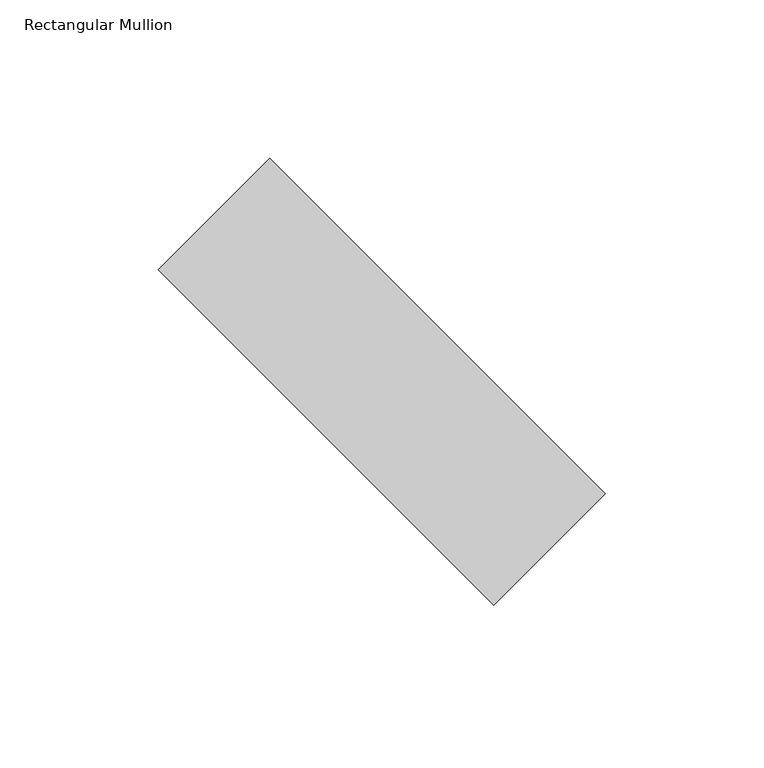
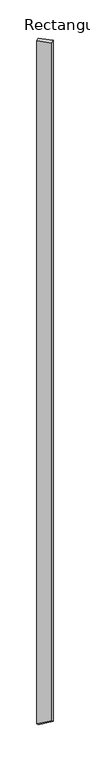
"""IFC4 building model written with IfcOpenShell, lengths in millimetres: member geometry, Rectangular Mullion : tilted mullions."""

from ifc_helpers import new_model, si_unit, origin, place, context, project, spatial, faceted_brep, source, transform, mapped, element, save


def rectangular_mullion_43ad61fc(model_context):
    return source(origin(), model_context, "Body", "Brep", [
        faceted_brep([(-35.3553391, 70.7106781, 0.0), (-70.7106781, 35.3553391, 0.0), (35.3553391, -70.7106781, 0.0), (70.7106781, -35.3553391, 0.0), (-35.3553391, 70.7106781, -8054.3955515), (-70.7106781, 35.3553391, -8009.3448964), (35.3553391, -70.7106781, -7944.276115), (70.7106781, -35.3553391, -7989.3267701)], [[[0, 1, 2, 3]], [[1, 0, 4, 5]], [[2, 1, 5, 6]], [[3, 2, 6, 7]], [[0, 3, 7, 4]], [[4, 7, 6, 5]]]),
    ])


if __name__ == "__main__":
    model = new_model("IFC4")
    model_context = context("Model", 3, world=origin())
    ifc_project = project(units=[si_unit("LENGTHUNIT", "METRE", prefix="MILLI")], contexts=[model_context])
    site = spatial("IfcSite", under=ifc_project)
    building = spatial("IfcBuilding", under=site)
    placement = place(None, origin())
    rectangular_mullion_shape = rectangular_mullion_43ad61fc(model_context)
    element("IfcMember", 1, ObjectType="Rectangular Mullion : tilted mullions", at=placement, inside=building, context=model_context, shape_type="MappedRepresentation", body=[
        mapped(rectangular_mullion_shape, transform((0.0, 0.0, 0.0), x_axis=(1.0, 0.0, 0.0), y_axis=(0.0, 1.0, 0.0), z_axis=(0.0, 0.0, 1.0))),
    ])
    save(model, "model.ifc")

# Revit data of these elements
# Type "Rectangular Mullion : tilted mullions"
#   built-in parameter 1007304 = 0.492126 (stored number, unit not read)
#   built-in parameter 1007301 = 0.082021 (stored number, unit not read)
#   built-in parameter 1007300 = 0.082021 (stored number, unit not read)
# Element 1 (IfcMember, "Rectangular Mullion : tilted mullions")
#   Materials on its faces: "Aluminum"
# Materials
#   "Aluminum": class "Metal", colour RGB 244 244 244, transparency 0, Description = "Aluminum 6061", Cost = 0
